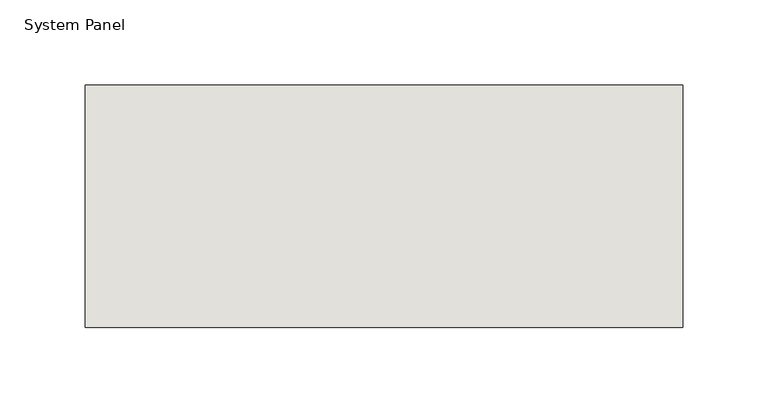
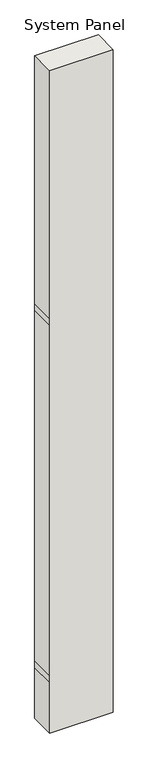
"""IFC4 building model written with IfcOpenShell, lengths in millimetres: wall geometry, System Panel : NLRS_21_CWP_hsb-vulling minerale wol 142 _gen_rsf."""

from ifc_helpers import new_model, si_unit, frame, origin, place, context, project, spatial, polyline, outline, extrude, source, transform, mapped, element, save


def system_panel_360973c8(model_context):
    return source(origin(), model_context, "Body", "SweptSolid", [
        extrude(outline(polyline([(0.0, -175.0000002), (0.0, 175.0000002), (295.0, 175.0000002), (333.0, 175.0000002), (2371.0, 175.0000002), (2409.0, 175.0000002), (3849.0, 175.0000002), (3849.0, -175.0000002), (2409.0, -175.0000002), (2371.0, -175.0000002), (333.0, -175.0000002), (295.0, -175.0000002), (0.0, -175.0000002)])), frame((0.0, -71.0, 0.0), z_axis=(0.0, 1.0, 0.0), x_axis=(0.0, 0.0, 1.0)), (0.0, 0.0, 1.0), 142.0),
    ])


if __name__ == "__main__":
    model = new_model("IFC4")
    model_context = context("Model", 3, world=origin())
    ifc_project = project(units=[si_unit("LENGTHUNIT", "METRE", prefix="MILLI")], contexts=[model_context])
    site = spatial("IfcSite", under=ifc_project)
    building = spatial("IfcBuilding", under=site)
    placement = place(None, origin())
    system_panel_shape = system_panel_360973c8(model_context)
    element("IfcWall", 1, ObjectType="System Panel : NLRS_21_CWP_hsb-vulling minerale wol 142 _gen_rsf", at=placement, inside=building, context=model_context, shape_type="MappedRepresentation", body=[
        mapped(system_panel_shape, transform((0.0, 0.0, 0.0), x_axis=(1.0, 0.0, 0.0), y_axis=(0.0, 1.0, 0.0), z_axis=(0.0, 0.0, 1.0))),
    ])
    save(model, "model.ifc")

# Revit data of these elements
# Type "System Panel : NLRS_21_CWP_hsb-vulling minerale wol 142 _gen_rsf"
#   Type IfcGUID = "07M7mRoiH1CR8m_RSKIwpC"
#   Assembly Code = "21.23"
#   IfcExportAs = "IfcWall"
# Element 1 (IfcWall, "System Panel : NLRS_21_CWP_hsb-vulling minerale wol 142 _gen_rsf")
#   Materials on its faces: "NLRS_m1_isolatie minerale wol_gen_rsf"
# Materials
#   "NLRS_m1_isolatie minerale wol_gen_rsf": class "M - Anorganische materialen", colour RGB 200 200 140, transparency 0, Keynote = "m1", Manufacturer = "Revit Standards Foundation", URL = "www.revitstandards.org", Description = "isolatie minerale wol", Cost = 0
